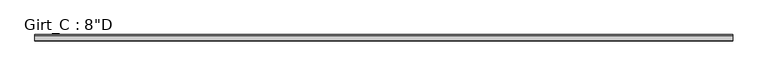
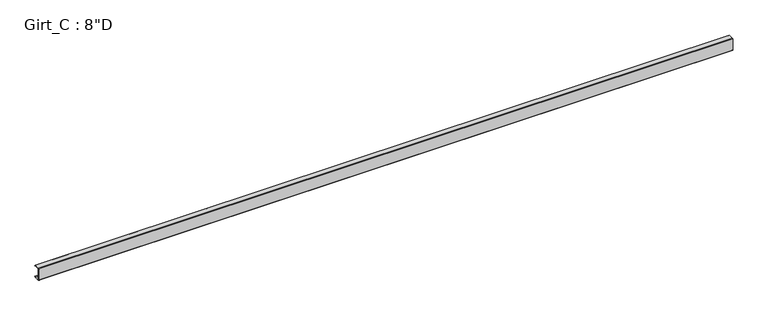
"""IFC4 building model written with IfcOpenShell, lengths in millimetres: beam geometry."""

from ifc_helpers import new_model, si_unit, point, frame, frame_2d, origin, place, context, project, spatial, polyline, circle_curve, trimmed, segment, composite_curve, outline, extrude, source, transform, mapped, element, save


def beam_95505e83(model_context):
    return source(origin(), model_context, "Body", "SweptSolid", [
        extrude(outline(composite_curve([segment(polyline([(87.5109375, 101.6), (99.7560415, 87.0068534), (97.6278742, 85.221109), (86.2154765, 98.821875), (3.3005807, 98.821875)]), True, "CONTINUOUS"), segment(trimmed(circle_curve(frame_2d((3.3741066, 96.8381931)), 1.9850441), [point((3.3005807, 98.821875))], [point((1.3890625, 96.8381931))], True, "CARTESIAN"), True, "CONTINUOUS"), segment(polyline([(1.3890625, 96.8381931), (1.3890625, -96.8389339)]), True, "CONTINUOUS"), segment(trimmed(circle_curve(frame_2d((3.3748024, -96.8389339)), 1.9857399), [point((1.3890625, -96.8389339))], [point((3.2694106, -98.821875))], True, "CARTESIAN"), True, "CONTINUOUS"), segment(polyline([(3.2694106, -98.821875), (86.2154765, -98.821875), (97.6510975, -85.1934327), (99.7792647, -86.979177), (87.5109375, -101.6), (3.3734375, -101.6)]), True, "CONTINUOUS"), segment(trimmed(circle_curve(frame_2d((3.3734375, -96.8375)), 4.7625), [point((3.3734375, -101.6))], [point((-1.3890625, -96.8375))], False, "CARTESIAN"), True, "CONTINUOUS"), segment(polyline([(-1.3890625, -96.8375), (-1.3890625, 96.8375)]), True, "CONTINUOUS"), segment(trimmed(circle_curve(frame_2d((3.3734375, 96.8375)), 4.7625), [point((-1.3890625, 96.8375))], [point((3.3734375, 101.6))], False, "CARTESIAN"), True, "CONTINUOUS"), segment(polyline([(3.3734375, 101.6), (87.5109375, 101.6)]), True, "CONTINUOUS")], self_intersect=False)), frame((-5621.3960998, 0.0, 0.0), z_axis=(1.0, 0.0, 0.0), x_axis=(0.0, 1.0, 0.0)), (0.0, 0.0, 1.0), 11076.8984495),
    ])


if __name__ == "__main__":
    model = new_model("IFC4")
    model_context = context("Model", 3, world=origin())
    ifc_project = project(units=[si_unit("LENGTHUNIT", "METRE", prefix="MILLI")], contexts=[model_context])
    site = spatial("IfcSite", under=ifc_project)
    building = spatial("IfcBuilding", under=site)
    placement = place(None, origin())
    beam_shape = beam_95505e83(model_context)
    element("IfcBeam", 1, ObjectType="Girt_C : 8\"D", at=placement, inside=building, context=model_context, shape_type="MappedRepresentation", body=[
        mapped(beam_shape, transform((0.0, 0.0, 0.0), x_axis=(1.0, 0.0, 0.0), y_axis=(0.0, 1.0, 0.0), z_axis=(0.0, 0.0, 1.0))),
    ])
    save(model, "model.ifc")

# Revit data of these elements
# Type "Girt_C : 8\"D"
#   half leg = 0' - 1 3/4"
#   Web_Thickness = 0' - 0 7/64"
#   Length [instance default] = 10' - 0"
#   Leg_1 = 0' - 3 1/2"
#   Height = 0' - 8"
#   Structural Material [instance default] = none
# Element 1 (IfcBeam, "Girt_C : 8\"D")
#   Structural Material = GALVANIZED 'CEE' SECTION (8.0x3.5C - SEE STRUCT. DWGS)
#   Materials on its faces: "GALVANIZED 'CEE' SECTION (8.0x3.5C - SEE STRUCT. DWGS)"
# Materials
#   "GALVANIZED 'CEE' SECTION (8.0x3.5C - SEE STRUCT. DWGS)": class "Metal", colour RGB 137 146 153, transparency 0, Description = "Steel, mill finish", Cost = 0
